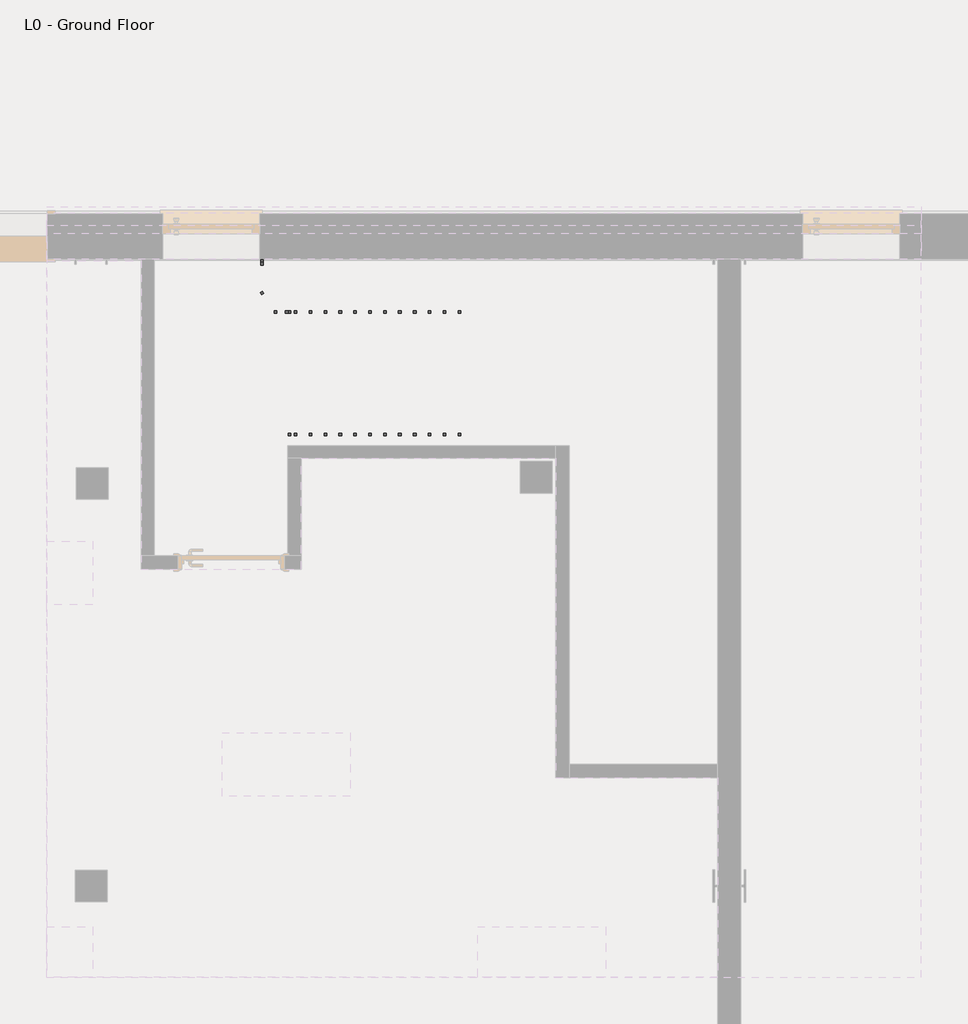
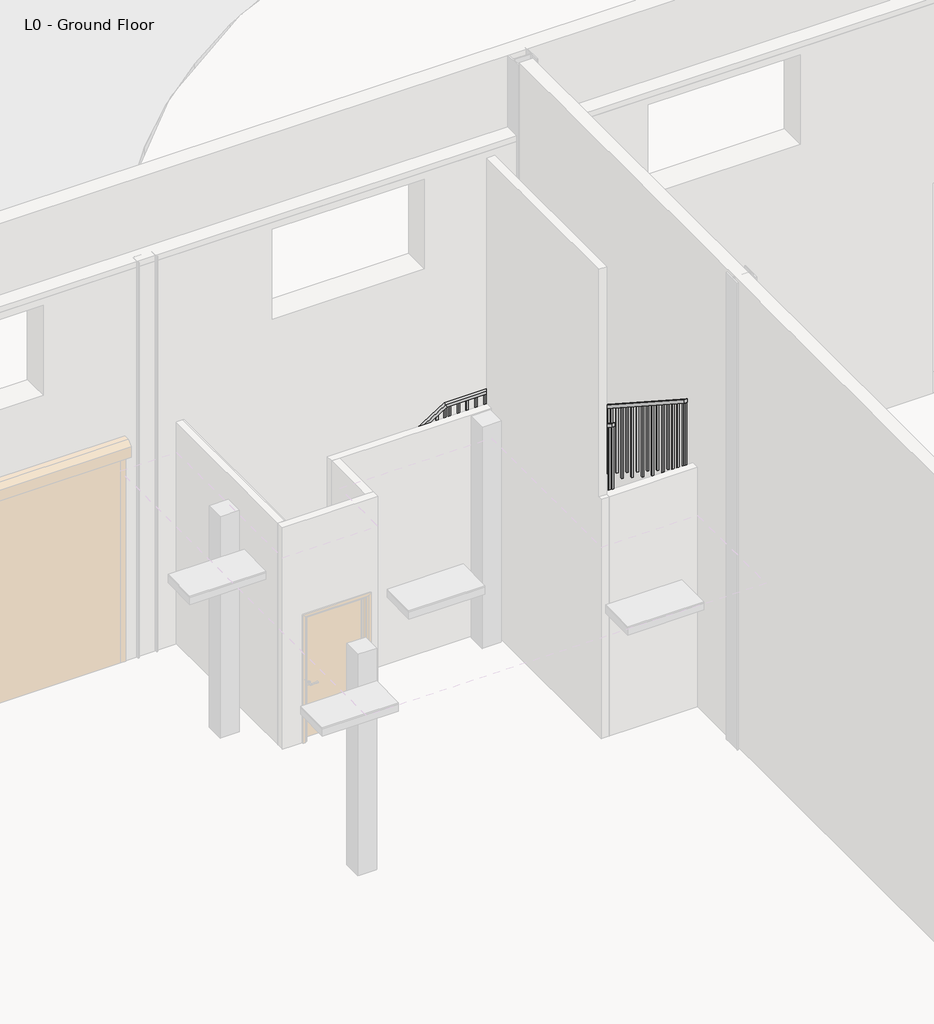
# One storey, part 11 of 14: 3 railings.
"""IFC4 building model written with IfcOpenShell, lengths in millimetres."""

from ifc_helpers import new_model, si_unit, frame, origin, place, context, project, spatial, polyline, outline, extrude, faceted_brep, element, save

model = new_model("IFC4")

# Units and contexts
model_context = context("Model", 3, world=origin())
ifc_project = project(units=[si_unit("LENGTHUNIT", "METRE", prefix="MILLI")], contexts=[model_context])

# Site, building, storey
site = spatial("IfcSite", under=ifc_project)
building = spatial("IfcBuilding", under=site)
storey = spatial("IfcBuildingStorey", under=building, Name="L0 - Ground Floor", Elevation=0.0)

# Railings
placement = place(None, origin())
element("IfcRailing", 1, ObjectType="1100mm", at=placement, inside=storey, context=model_context, shape_type="SolidModel", body=[
    faceted_brep([(6712.9446543, 5212.4222729, 1286.5612648), (6712.9446543, 5212.4222729, 1227.4016553), (6712.9446543, 5162.4222729, 1227.4016553), (6712.9446543, 5162.4222729, 1286.5612648), (9292.9446543, 5212.4222729, 2918.1818182), (9307.4282868, 5212.4222729, 2868.1818182), (9307.4282868, 5162.4222729, 2868.1818182), (9292.9446543, 5162.4222729, 2918.1818182), (9390.9278057, 5212.4222729, 2918.1818182), (9440.9278057, 5212.4222729, 2868.1818182), (9440.9278057, 5162.4222729, 2868.1818182), (9390.9278057, 5162.4222729, 2918.1818182), (9390.9278057, 5212.4222729, 3148.4415584), (9440.9278057, 5212.4222729, 3098.4415584), (9440.9278057, 5162.4222729, 3098.4415584), (9390.9278057, 5162.4222729, 3148.4415584), (9515.9278057, 5212.4222729, 3148.4415584), (9515.9278057, 5212.4222729, 3098.4415584), (9465.9278057, 5162.4222729, 3098.4415584), (9465.9278057, 5162.4222729, 3148.4415584), (9515.9278057, 5087.4222729, 3148.4415584), (9515.9278057, 5072.6126873, 3098.4415584), (9465.9278057, 5072.6126873, 3098.4415584), (9465.9278057, 5087.4222729, 3148.4415584), (9515.9278057, 2082.0222729, 5100.0), (9465.9278057, 2082.0222729, 5100.0), (9465.9278057, 2082.0222729, 5040.383386), (9515.9278057, 2082.0222729, 5040.383386)], [[[0, 1, 2, 3]], [[1, 0, 4, 5]], [[2, 1, 5, 6]], [[3, 2, 6, 7]], [[0, 3, 7, 4]], [[5, 4, 8, 9]], [[6, 5, 9, 10]], [[7, 6, 10, 11]], [[4, 7, 11, 8]], [[9, 8, 12, 13]], [[10, 9, 13, 14]], [[11, 10, 14, 15]], [[8, 11, 15, 12]], [[13, 12, 16, 17]], [[14, 13, 17, 18]], [[15, 14, 18, 19]], [[12, 15, 19, 16]], [[17, 16, 20, 21]], [[18, 17, 21, 22]], [[19, 18, 22, 23]], [[16, 19, 23, 20]], [[24, 25, 26, 27]], [[21, 20, 24, 27]], [[22, 21, 27, 26]], [[23, 22, 26, 25]], [[20, 23, 25, 24]]]),
    extrude(outline(polyline([(2189.9222729, 4970.3184509), (2189.9222729, 3818.1818182), (2164.9222729, 3818.1818182), (2164.9222729, 4986.5522172), (2189.9222729, 4970.3184509)])), frame((9478.4278057, 0.0, 0.0), z_axis=(1.0, 0.0, 0.0), x_axis=(0.0, 1.0, 0.0)), (0.0, 0.0, 1.0), 25.0),
    extrude(outline(polyline([(2329.9222729, 4879.40936), (2329.9222729, 3818.1818182), (2304.9222729, 3818.1818182), (2304.9222729, 4895.6431263), (2329.9222729, 4879.40936)])), frame((9478.4278057, 0.0, 0.0), z_axis=(1.0, 0.0, 0.0), x_axis=(0.0, 1.0, 0.0)), (0.0, 0.0, 1.0), 25.0),
    extrude(outline(polyline([(2469.9222729, 4788.5002691), (2469.9222729, 3636.3636364), (2444.9222729, 3636.3636364), (2444.9222729, 4804.7340354), (2469.9222729, 4788.5002691)])), frame((9478.4278057, 0.0, 0.0), z_axis=(1.0, 0.0, 0.0), x_axis=(0.0, 1.0, 0.0)), (0.0, 0.0, 1.0), 25.0),
    extrude(outline(polyline([(2609.9222729, 4697.5911782), (2609.9222729, 3636.3636364), (2584.9222729, 3636.3636364), (2584.9222729, 4713.8249444), (2609.9222729, 4697.5911782)])), frame((9478.4278057, 0.0, 0.0), z_axis=(1.0, 0.0, 0.0), x_axis=(0.0, 1.0, 0.0)), (0.0, 0.0, 1.0), 25.0),
    extrude(outline(polyline([(2749.9222729, 4606.6820873), (2749.9222729, 3454.5454545), (2724.9222729, 3454.5454545), (2724.9222729, 4622.9158535), (2749.9222729, 4606.6820873)])), frame((9478.4278057, 0.0, 0.0), z_axis=(1.0, 0.0, 0.0), x_axis=(0.0, 1.0, 0.0)), (0.0, 0.0, 1.0), 25.0),
    extrude(outline(polyline([(2889.9222729, 4515.7729964), (2889.9222729, 3454.5454545), (2864.9222729, 3454.5454545), (2864.9222729, 4532.0067626), (2889.9222729, 4515.7729964)])), frame((9478.4278057, 0.0, 0.0), z_axis=(1.0, 0.0, 0.0), x_axis=(0.0, 1.0, 0.0)), (0.0, 0.0, 1.0), 25.0),
    extrude(outline(polyline([(3029.9222729, 4424.8639055), (3029.9222729, 3272.7272727), (3004.9222729, 3272.7272727), (3004.9222729, 4441.0976717), (3029.9222729, 4424.8639055)])), frame((9478.4278057, 0.0, 0.0), z_axis=(1.0, 0.0, 0.0), x_axis=(0.0, 1.0, 0.0)), (0.0, 0.0, 1.0), 25.0),
    extrude(outline(polyline([(3169.9222729, 4333.9548146), (3169.9222729, 3272.7272727), (3144.9222729, 3272.7272727), (3144.9222729, 4350.1885808), (3169.9222729, 4333.9548146)])), frame((9478.4278057, 0.0, 0.0), z_axis=(1.0, 0.0, 0.0), x_axis=(0.0, 1.0, 0.0)), (0.0, 0.0, 1.0), 25.0),
    extrude(outline(polyline([(3309.9222729, 4243.0457237), (3309.9222729, 3090.9090909), (3284.9222729, 3090.9090909), (3284.9222729, 4259.2794899), (3309.9222729, 4243.0457237)])), frame((9478.4278057, 0.0, 0.0), z_axis=(1.0, 0.0, 0.0), x_axis=(0.0, 1.0, 0.0)), (0.0, 0.0, 1.0), 25.0),
    extrude(outline(polyline([(3449.9222729, 4152.1366328), (3449.9222729, 3090.9090909), (3424.9222729, 3090.9090909), (3424.9222729, 4168.370399), (3449.9222729, 4152.1366328)])), frame((9478.4278057, 0.0, 0.0), z_axis=(1.0, 0.0, 0.0), x_axis=(0.0, 1.0, 0.0)), (0.0, 0.0, 1.0), 25.0),
    extrude(outline(polyline([(3589.9222729, 4061.2275418), (3589.9222729, 2909.0909091), (3564.9222729, 2909.0909091), (3564.9222729, 4077.4613081), (3589.9222729, 4061.2275418)])), frame((9478.4278057, 0.0, 0.0), z_axis=(1.0, 0.0, 0.0), x_axis=(0.0, 1.0, 0.0)), (0.0, 0.0, 1.0), 25.0),
    extrude(outline(polyline([(3729.9222729, 3970.3184509), (3729.9222729, 2909.0909091), (3704.9222729, 2909.0909091), (3704.9222729, 3986.5522172), (3729.9222729, 3970.3184509)])), frame((9478.4278057, 0.0, 0.0), z_axis=(1.0, 0.0, 0.0), x_axis=(0.0, 1.0, 0.0)), (0.0, 0.0, 1.0), 25.0),
    extrude(outline(polyline([(3869.9222729, 3879.40936), (3869.9222729, 2727.2727273), (3844.9222729, 2727.2727273), (3844.9222729, 3895.6431263), (3869.9222729, 3879.40936)])), frame((9478.4278057, 0.0, 0.0), z_axis=(1.0, 0.0, 0.0), x_axis=(0.0, 1.0, 0.0)), (0.0, 0.0, 1.0), 25.0),
    extrude(outline(polyline([(4009.9222729, 3788.5002691), (4009.9222729, 2727.2727273), (3984.9222729, 2727.2727273), (3984.9222729, 3804.7340354), (4009.9222729, 3788.5002691)])), frame((9478.4278057, 0.0, 0.0), z_axis=(1.0, 0.0, 0.0), x_axis=(0.0, 1.0, 0.0)), (0.0, 0.0, 1.0), 25.0),
    extrude(outline(polyline([(4149.9222729, 3697.5911782), (4149.9222729, 2545.4545455), (4124.9222729, 2545.4545455), (4124.9222729, 3713.8249444), (4149.9222729, 3697.5911782)])), frame((9478.4278057, 0.0, 0.0), z_axis=(1.0, 0.0, 0.0), x_axis=(0.0, 1.0, 0.0)), (0.0, 0.0, 1.0), 25.0),
    extrude(outline(polyline([(4289.9222729, 3606.6820873), (4289.9222729, 2545.4545455), (4264.9222729, 2545.4545455), (4264.9222729, 3622.9158535), (4289.9222729, 3606.6820873)])), frame((9478.4278057, 0.0, 0.0), z_axis=(1.0, 0.0, 0.0), x_axis=(0.0, 1.0, 0.0)), (0.0, 0.0, 1.0), 25.0),
    extrude(outline(polyline([(4429.9222729, 3515.7729964), (4429.9222729, 2363.6363636), (4404.9222729, 2363.6363636), (4404.9222729, 3532.0067626), (4429.9222729, 3515.7729964)])), frame((9478.4278057, 0.0, 0.0), z_axis=(1.0, 0.0, 0.0), x_axis=(0.0, 1.0, 0.0)), (0.0, 0.0, 1.0), 25.0),
    extrude(outline(polyline([(4569.9222729, 3424.8639055), (4569.9222729, 2363.6363636), (4544.9222729, 2363.6363636), (4544.9222729, 3441.0976717), (4569.9222729, 3424.8639055)])), frame((9478.4278057, 0.0, 0.0), z_axis=(1.0, 0.0, 0.0), x_axis=(0.0, 1.0, 0.0)), (0.0, 0.0, 1.0), 25.0),
    extrude(outline(polyline([(4709.9222729, 3333.9548146), (4709.9222729, 2181.8181818), (4684.9222729, 2181.8181818), (4684.9222729, 3350.1885808), (4709.9222729, 3333.9548146)])), frame((9478.4278057, 0.0, 0.0), z_axis=(1.0, 0.0, 0.0), x_axis=(0.0, 1.0, 0.0)), (0.0, 0.0, 1.0), 25.0),
    extrude(outline(polyline([(4849.9222729, 3243.0457237), (4849.9222729, 2181.8181818), (4824.9222729, 2181.8181818), (4824.9222729, 3259.2794899), (4849.9222729, 3243.0457237)])), frame((9478.4278057, 0.0, 0.0), z_axis=(1.0, 0.0, 0.0), x_axis=(0.0, 1.0, 0.0)), (0.0, 0.0, 1.0), 25.0),
    extrude(outline(polyline([(4989.9222729, 3152.1366328), (4989.9222729, 2000.0), (4964.9222729, 2000.0), (4964.9222729, 3168.370399), (4989.9222729, 3152.1366328)])), frame((9478.4278057, 0.0, 0.0), z_axis=(1.0, 0.0, 0.0), x_axis=(0.0, 1.0, 0.0)), (0.0, 0.0, 1.0), 25.0),
    extrude(outline(polyline([(9478.4278057, 5129.9222729), (9503.4278057, 5129.9222729), (9503.4278057, 5104.9222729), (9478.4278057, 5104.9222729), (9478.4278057, 5129.9222729)])), frame((0.0, 0.0, 2000.0), z_axis=(0.0, 0.0, 1.0), x_axis=(1.0, 0.0, 0.0)), (0.0, 0.0, 1.0), 1098.4415584),
    extrude(outline(polyline([(9350.4446543, 5174.9222729), (9350.4446543, 5199.9222729), (9375.4446543, 5199.9222729), (9375.4446543, 5174.9222729), (9350.4446543, 5174.9222729)])), frame((0.0, 0.0, 1818.1818182), z_axis=(0.0, 0.0, 1.0), x_axis=(1.0, 0.0, 0.0)), (0.0, 0.0, 1.0), 1050.0),
    extrude(outline(polyline([(2768.9036316, 9150.4446543), (1636.3636364, 9150.4446543), (1636.3636364, 9175.4446543), (2784.7139083, 9175.4446543), (2768.9036316, 9150.4446543)])), frame((0.0, 5174.9222729, 0.0), z_axis=(0.0, 1.0, 0.0), x_axis=(0.0, 0.0, 1.0)), (0.0, 0.0, 1.0), 25.0),
    extrude(outline(polyline([(2680.3660822, 9010.4446543), (1636.3636364, 9010.4446543), (1636.3636364, 9035.4446543), (2696.1763589, 9035.4446543), (2680.3660822, 9010.4446543)])), frame((0.0, 5174.9222729, 0.0), z_axis=(0.0, 1.0, 0.0), x_axis=(0.0, 0.0, 1.0)), (0.0, 0.0, 1.0), 25.0),
    extrude(outline(polyline([(2591.8285328, 8870.4446543), (1454.5454545, 8870.4446543), (1454.5454545, 8895.4446543), (2607.6388095, 8895.4446543), (2591.8285328, 8870.4446543)])), frame((0.0, 5174.9222729, 0.0), z_axis=(0.0, 1.0, 0.0), x_axis=(0.0, 0.0, 1.0)), (0.0, 0.0, 1.0), 25.0),
    extrude(outline(polyline([(2503.2909834, 8730.4446543), (1454.5454545, 8730.4446543), (1454.5454545, 8755.4446543), (2519.1012601, 8755.4446543), (2503.2909834, 8730.4446543)])), frame((0.0, 5174.9222729, 0.0), z_axis=(0.0, 1.0, 0.0), x_axis=(0.0, 0.0, 1.0)), (0.0, 0.0, 1.0), 25.0),
    extrude(outline(polyline([(2414.753434, 8590.4446543), (1272.7272727, 8590.4446543), (1272.7272727, 8615.4446543), (2430.5637107, 8615.4446543), (2414.753434, 8590.4446543)])), frame((0.0, 5174.9222729, 0.0), z_axis=(0.0, 1.0, 0.0), x_axis=(0.0, 0.0, 1.0)), (0.0, 0.0, 1.0), 25.0),
    extrude(outline(polyline([(2326.2158846, 8450.4446543), (1272.7272727, 8450.4446543), (1272.7272727, 8475.4446543), (2342.0261613, 8475.4446543), (2326.2158846, 8450.4446543)])), frame((0.0, 5174.9222729, 0.0), z_axis=(0.0, 1.0, 0.0), x_axis=(0.0, 0.0, 1.0)), (0.0, 0.0, 1.0), 25.0),
    extrude(outline(polyline([(2237.6783352, 8310.4446543), (1090.9090909, 8310.4446543), (1090.9090909, 8335.4446543), (2253.4886119, 8335.4446543), (2237.6783352, 8310.4446543)])), frame((0.0, 5174.9222729, 0.0), z_axis=(0.0, 1.0, 0.0), x_axis=(0.0, 0.0, 1.0)), (0.0, 0.0, 1.0), 25.0),
    extrude(outline(polyline([(2149.1407858, 8170.4446543), (1090.9090909, 8170.4446543), (1090.9090909, 8195.4446543), (2164.9510624, 8195.4446543), (2149.1407858, 8170.4446543)])), frame((0.0, 5174.9222729, 0.0), z_axis=(0.0, 1.0, 0.0), x_axis=(0.0, 0.0, 1.0)), (0.0, 0.0, 1.0), 25.0),
    extrude(outline(polyline([(2060.6032364, 8030.4446543), (909.0909091, 8030.4446543), (909.0909091, 8055.4446543), (2076.413513, 8055.4446543), (2060.6032364, 8030.4446543)])), frame((0.0, 5174.9222729, 0.0), z_axis=(0.0, 1.0, 0.0), x_axis=(0.0, 0.0, 1.0)), (0.0, 0.0, 1.0), 25.0),
    extrude(outline(polyline([(1972.065687, 7890.4446543), (909.0909091, 7890.4446543), (909.0909091, 7915.4446543), (1987.8759636, 7915.4446543), (1972.065687, 7890.4446543)])), frame((0.0, 5174.9222729, 0.0), z_axis=(0.0, 1.0, 0.0), x_axis=(0.0, 0.0, 1.0)), (0.0, 0.0, 1.0), 25.0),
    extrude(outline(polyline([(1883.5281375, 7750.4446543), (727.2727273, 7750.4446543), (727.2727273, 7775.4446543), (1899.3384142, 7775.4446543), (1883.5281375, 7750.4446543)])), frame((0.0, 5174.9222729, 0.0), z_axis=(0.0, 1.0, 0.0), x_axis=(0.0, 0.0, 1.0)), (0.0, 0.0, 1.0), 25.0),
    extrude(outline(polyline([(1794.9905881, 7610.4446543), (727.2727273, 7610.4446543), (727.2727273, 7635.4446543), (1810.8008648, 7635.4446543), (1794.9905881, 7610.4446543)])), frame((0.0, 5174.9222729, 0.0), z_axis=(0.0, 1.0, 0.0), x_axis=(0.0, 0.0, 1.0)), (0.0, 0.0, 1.0), 25.0),
    extrude(outline(polyline([(1706.4530387, 7470.4446543), (545.4545455, 7470.4446543), (545.4545455, 7495.4446543), (1722.2633154, 7495.4446543), (1706.4530387, 7470.4446543)])), frame((0.0, 5174.9222729, 0.0), z_axis=(0.0, 1.0, 0.0), x_axis=(0.0, 0.0, 1.0)), (0.0, 0.0, 1.0), 25.0),
    extrude(outline(polyline([(1617.9154893, 7330.4446543), (545.4545455, 7330.4446543), (545.4545455, 7355.4446543), (1633.725766, 7355.4446543), (1617.9154893, 7330.4446543)])), frame((0.0, 5174.9222729, 0.0), z_axis=(0.0, 1.0, 0.0), x_axis=(0.0, 0.0, 1.0)), (0.0, 0.0, 1.0), 25.0),
    extrude(outline(polyline([(1529.3779399, 7190.4446543), (363.6363636, 7190.4446543), (363.6363636, 7215.4446543), (1545.1882166, 7215.4446543), (1529.3779399, 7190.4446543)])), frame((0.0, 5174.9222729, 0.0), z_axis=(0.0, 1.0, 0.0), x_axis=(0.0, 0.0, 1.0)), (0.0, 0.0, 1.0), 25.0),
    extrude(outline(polyline([(1440.8403905, 7050.4446543), (363.6363636, 7050.4446543), (363.6363636, 7075.4446543), (1456.6506672, 7075.4446543), (1440.8403905, 7050.4446543)])), frame((0.0, 5174.9222729, 0.0), z_axis=(0.0, 1.0, 0.0), x_axis=(0.0, 0.0, 1.0)), (0.0, 0.0, 1.0), 25.0),
    extrude(outline(polyline([(1352.3028411, 6910.4446543), (181.8181818, 6910.4446543), (181.8181818, 6935.4446543), (1368.1131178, 6935.4446543), (1352.3028411, 6910.4446543)])), frame((0.0, 5174.9222729, 0.0), z_axis=(0.0, 1.0, 0.0), x_axis=(0.0, 0.0, 1.0)), (0.0, 0.0, 1.0), 25.0),
    extrude(outline(polyline([(1263.7652917, 6770.4446543), (181.8181818, 6770.4446543), (181.8181818, 6795.4446543), (1279.5755684, 6795.4446543), (1263.7652917, 6770.4446543)])), frame((0.0, 5174.9222729, 0.0), z_axis=(0.0, 1.0, 0.0), x_axis=(0.0, 0.0, 1.0)), (0.0, 0.0, 1.0), 25.0),
    extrude(outline(polyline([(9478.4278057, 5199.9222729), (9503.4278057, 5199.9222729), (9503.4278057, 5174.9222729), (9478.4278057, 5174.9222729), (9478.4278057, 5199.9222729)])), frame((0.0, 0.0, 1818.1818182), z_axis=(0.0, 0.0, 1.0), x_axis=(1.0, 0.0, 0.0)), (0.0, 0.0, 1.0), 1280.2597403),
    extrude(outline(polyline([(2851.1170704, 9280.4446543), (1818.1818182, 9280.4446543), (1818.1818182, 9305.4446543), (2866.927347, 9305.4446543), (2851.1170704, 9280.4446543)])), frame((0.0, 5174.9222729, 0.0), z_axis=(0.0, 1.0, 0.0), x_axis=(0.0, 0.0, 1.0)), (0.0, 0.0, 1.0), 25.0),
    extrude(outline(polyline([(2107.0222729, 5024.1496198), (2107.0222729, 3818.1818182), (2082.0222729, 3818.1818182), (2082.0222729, 5040.383386), (2107.0222729, 5024.1496198)])), frame((9478.4278057, 0.0, 0.0), z_axis=(1.0, 0.0, 0.0), x_axis=(0.0, 1.0, 0.0)), (0.0, 0.0, 1.0), 25.0),
    extrude(outline(polyline([(1227.4016553, 6712.9446543), (181.8181818, 6712.9446543), (181.8181818, 6737.9446543), (1243.211932, 6737.9446543), (1227.4016553, 6712.9446543)])), frame((0.0, 5174.9222729, 0.0), z_axis=(0.0, 1.0, 0.0), x_axis=(0.0, 0.0, 1.0)), (0.0, 0.0, 1.0), 25.0),
])
element("IfcRailing", 2, ObjectType="1100mm", at=placement, inside=storey, context=model_context, shape_type="SolidModel", body=[
    faceted_brep([(6712.9446543, 6361.6222729, 1286.5612648), (6712.9446543, 6361.6222729, 1227.4016553), (6712.9446543, 6311.6222729, 1227.4016553), (6712.9446543, 6311.6222729, 1286.5612648), (9292.9446543, 6361.6222729, 2918.1818182), (9307.4282868, 6361.6222729, 2868.1818182), (9307.4282868, 6311.6222729, 2868.1818182), (9292.9446543, 6311.6222729, 2918.1818182), (10665.1278057, 6361.6222729, 2918.1818182), (10665.1278057, 6361.6222729, 2868.1818182), (10615.1278057, 6311.6222729, 2868.1818182), (10615.1278057, 6311.6222729, 2918.1818182), (10665.1278057, 5442.0222729, 2918.1818182), (10665.1278057, 5427.2126873, 2868.1818182), (10615.1278057, 5427.2126873, 2868.1818182), (10615.1278057, 5442.0222729, 2918.1818182), (10665.1278057, 2082.0222729, 5100.0), (10615.1278057, 2082.0222729, 5100.0), (10615.1278057, 2082.0222729, 5040.383386), (10665.1278057, 2082.0222729, 5040.383386)], [[[0, 1, 2, 3]], [[1, 0, 4, 5]], [[2, 1, 5, 6]], [[3, 2, 6, 7]], [[0, 3, 7, 4]], [[5, 4, 8, 9]], [[6, 5, 9, 10]], [[7, 6, 10, 11]], [[4, 7, 11, 8]], [[9, 8, 12, 13]], [[10, 9, 13, 14]], [[11, 10, 14, 15]], [[8, 11, 15, 12]], [[16, 17, 18, 19]], [[13, 12, 16, 19]], [[14, 13, 19, 18]], [[15, 14, 18, 17]], [[12, 15, 17, 16]]]),
    extrude(outline(polyline([(2164.5222729, 3818.1818182), (2139.5222729, 3818.1818182), (2139.5222729, 5003.0457237), (2164.5222729, 4986.8119574), (2164.5222729, 3818.1818182)])), frame((10627.6278057, 0.0, 0.0), z_axis=(1.0, 0.0, 0.0), x_axis=(0.0, 1.0, 0.0)), (0.0, 0.0, 1.0), 25.0),
    extrude(outline(polyline([(2304.5222729, 3818.1818182), (2279.5222729, 3818.1818182), (2279.5222729, 4912.1366328), (2304.5222729, 4895.9028665), (2304.5222729, 3818.1818182)])), frame((10627.6278057, 0.0, 0.0), z_axis=(1.0, 0.0, 0.0), x_axis=(0.0, 1.0, 0.0)), (0.0, 0.0, 1.0), 25.0),
    extrude(outline(polyline([(2444.5222729, 3636.3636364), (2419.5222729, 3636.3636364), (2419.5222729, 4821.2275418), (2444.5222729, 4804.9937756), (2444.5222729, 3636.3636364)])), frame((10627.6278057, 0.0, 0.0), z_axis=(1.0, 0.0, 0.0), x_axis=(0.0, 1.0, 0.0)), (0.0, 0.0, 1.0), 25.0),
    extrude(outline(polyline([(2584.5222729, 3636.3636364), (2559.5222729, 3636.3636364), (2559.5222729, 4730.3184509), (2584.5222729, 4714.0846847), (2584.5222729, 3636.3636364)])), frame((10627.6278057, 0.0, 0.0), z_axis=(1.0, 0.0, 0.0), x_axis=(0.0, 1.0, 0.0)), (0.0, 0.0, 1.0), 25.0),
    extrude(outline(polyline([(2724.5222729, 3454.5454545), (2699.5222729, 3454.5454545), (2699.5222729, 4639.40936), (2724.5222729, 4623.1755938), (2724.5222729, 3454.5454545)])), frame((10627.6278057, 0.0, 0.0), z_axis=(1.0, 0.0, 0.0), x_axis=(0.0, 1.0, 0.0)), (0.0, 0.0, 1.0), 25.0),
    extrude(outline(polyline([(2864.5222729, 3454.5454545), (2839.5222729, 3454.5454545), (2839.5222729, 4548.5002691), (2864.5222729, 4532.2665029), (2864.5222729, 3454.5454545)])), frame((10627.6278057, 0.0, 0.0), z_axis=(1.0, 0.0, 0.0), x_axis=(0.0, 1.0, 0.0)), (0.0, 0.0, 1.0), 25.0),
    extrude(outline(polyline([(3004.5222729, 3272.7272727), (2979.5222729, 3272.7272727), (2979.5222729, 4457.5911782), (3004.5222729, 4441.357412), (3004.5222729, 3272.7272727)])), frame((10627.6278057, 0.0, 0.0), z_axis=(1.0, 0.0, 0.0), x_axis=(0.0, 1.0, 0.0)), (0.0, 0.0, 1.0), 25.0),
    extrude(outline(polyline([(3144.5222729, 3272.7272727), (3119.5222729, 3272.7272727), (3119.5222729, 4366.6820873), (3144.5222729, 4350.4483211), (3144.5222729, 3272.7272727)])), frame((10627.6278057, 0.0, 0.0), z_axis=(1.0, 0.0, 0.0), x_axis=(0.0, 1.0, 0.0)), (0.0, 0.0, 1.0), 25.0),
    extrude(outline(polyline([(3284.5222729, 3090.9090909), (3259.5222729, 3090.9090909), (3259.5222729, 4275.7729964), (3284.5222729, 4259.5392302), (3284.5222729, 3090.9090909)])), frame((10627.6278057, 0.0, 0.0), z_axis=(1.0, 0.0, 0.0), x_axis=(0.0, 1.0, 0.0)), (0.0, 0.0, 1.0), 25.0),
    extrude(outline(polyline([(3424.5222729, 3090.9090909), (3399.5222729, 3090.9090909), (3399.5222729, 4184.8639055), (3424.5222729, 4168.6301392), (3424.5222729, 3090.9090909)])), frame((10627.6278057, 0.0, 0.0), z_axis=(1.0, 0.0, 0.0), x_axis=(0.0, 1.0, 0.0)), (0.0, 0.0, 1.0), 25.0),
    extrude(outline(polyline([(3564.5222729, 2909.0909091), (3539.5222729, 2909.0909091), (3539.5222729, 4093.9548146), (3564.5222729, 4077.7210483), (3564.5222729, 2909.0909091)])), frame((10627.6278057, 0.0, 0.0), z_axis=(1.0, 0.0, 0.0), x_axis=(0.0, 1.0, 0.0)), (0.0, 0.0, 1.0), 25.0),
    extrude(outline(polyline([(3704.5222729, 2909.0909091), (3679.5222729, 2909.0909091), (3679.5222729, 4003.0457237), (3704.5222729, 3986.8119574), (3704.5222729, 2909.0909091)])), frame((10627.6278057, 0.0, 0.0), z_axis=(1.0, 0.0, 0.0), x_axis=(0.0, 1.0, 0.0)), (0.0, 0.0, 1.0), 25.0),
    extrude(outline(polyline([(3844.5222729, 2727.2727273), (3819.5222729, 2727.2727273), (3819.5222729, 3912.1366328), (3844.5222729, 3895.9028665), (3844.5222729, 2727.2727273)])), frame((10627.6278057, 0.0, 0.0), z_axis=(1.0, 0.0, 0.0), x_axis=(0.0, 1.0, 0.0)), (0.0, 0.0, 1.0), 25.0),
    extrude(outline(polyline([(3984.5222729, 2727.2727273), (3959.5222729, 2727.2727273), (3959.5222729, 3821.2275418), (3984.5222729, 3804.9937756), (3984.5222729, 2727.2727273)])), frame((10627.6278057, 0.0, 0.0), z_axis=(1.0, 0.0, 0.0), x_axis=(0.0, 1.0, 0.0)), (0.0, 0.0, 1.0), 25.0),
    extrude(outline(polyline([(4124.5222729, 2545.4545455), (4099.5222729, 2545.4545455), (4099.5222729, 3730.3184509), (4124.5222729, 3714.0846847), (4124.5222729, 2545.4545455)])), frame((10627.6278057, 0.0, 0.0), z_axis=(1.0, 0.0, 0.0), x_axis=(0.0, 1.0, 0.0)), (0.0, 0.0, 1.0), 25.0),
    extrude(outline(polyline([(4264.5222729, 2545.4545455), (4239.5222729, 2545.4545455), (4239.5222729, 3639.40936), (4264.5222729, 3623.1755938), (4264.5222729, 2545.4545455)])), frame((10627.6278057, 0.0, 0.0), z_axis=(1.0, 0.0, 0.0), x_axis=(0.0, 1.0, 0.0)), (0.0, 0.0, 1.0), 25.0),
    extrude(outline(polyline([(4404.5222729, 2363.6363636), (4379.5222729, 2363.6363636), (4379.5222729, 3548.5002691), (4404.5222729, 3532.2665029), (4404.5222729, 2363.6363636)])), frame((10627.6278057, 0.0, 0.0), z_axis=(1.0, 0.0, 0.0), x_axis=(0.0, 1.0, 0.0)), (0.0, 0.0, 1.0), 25.0),
    extrude(outline(polyline([(4544.5222729, 2363.6363636), (4519.5222729, 2363.6363636), (4519.5222729, 3457.5911782), (4544.5222729, 3441.357412), (4544.5222729, 2363.6363636)])), frame((10627.6278057, 0.0, 0.0), z_axis=(1.0, 0.0, 0.0), x_axis=(0.0, 1.0, 0.0)), (0.0, 0.0, 1.0), 25.0),
    extrude(outline(polyline([(4684.5222729, 2181.8181818), (4659.5222729, 2181.8181818), (4659.5222729, 3366.6820873), (4684.5222729, 3350.4483211), (4684.5222729, 2181.8181818)])), frame((10627.6278057, 0.0, 0.0), z_axis=(1.0, 0.0, 0.0), x_axis=(0.0, 1.0, 0.0)), (0.0, 0.0, 1.0), 25.0),
    extrude(outline(polyline([(4824.5222729, 2181.8181818), (4799.5222729, 2181.8181818), (4799.5222729, 3275.7729964), (4824.5222729, 3259.5392302), (4824.5222729, 2181.8181818)])), frame((10627.6278057, 0.0, 0.0), z_axis=(1.0, 0.0, 0.0), x_axis=(0.0, 1.0, 0.0)), (0.0, 0.0, 1.0), 25.0),
    extrude(outline(polyline([(4964.5222729, 2000.0), (4939.5222729, 2000.0), (4939.5222729, 3184.8639055), (4964.5222729, 3168.6301392), (4964.5222729, 2000.0)])), frame((10627.6278057, 0.0, 0.0), z_axis=(1.0, 0.0, 0.0), x_axis=(0.0, 1.0, 0.0)), (0.0, 0.0, 1.0), 25.0),
    extrude(outline(polyline([(5104.5222729, 2000.0), (5079.5222729, 2000.0), (5079.5222729, 3093.9548146), (5104.5222729, 3077.7210483), (5104.5222729, 2000.0)])), frame((10627.6278057, 0.0, 0.0), z_axis=(1.0, 0.0, 0.0), x_axis=(0.0, 1.0, 0.0)), (0.0, 0.0, 1.0), 25.0),
    extrude(outline(polyline([(5244.5222729, 1818.1818182), (5219.5222729, 1818.1818182), (5219.5222729, 3003.0457237), (5244.5222729, 2986.8119574), (5244.5222729, 1818.1818182)])), frame((10627.6278057, 0.0, 0.0), z_axis=(1.0, 0.0, 0.0), x_axis=(0.0, 1.0, 0.0)), (0.0, 0.0, 1.0), 25.0),
    extrude(outline(polyline([(5384.5222729, 1818.1818182), (5359.5222729, 1818.1818182), (5359.5222729, 2912.1366328), (5384.5222729, 2895.9028665), (5384.5222729, 1818.1818182)])), frame((10627.6278057, 0.0, 0.0), z_axis=(1.0, 0.0, 0.0), x_axis=(0.0, 1.0, 0.0)), (0.0, 0.0, 1.0), 25.0),
    extrude(outline(polyline([(10652.6278057, 5579.1222729), (10652.6278057, 5554.1222729), (10627.6278057, 5554.1222729), (10627.6278057, 5579.1222729), (10652.6278057, 5579.1222729)])), frame((0.0, 0.0, 1818.1818182), z_axis=(0.0, 0.0, 1.0), x_axis=(1.0, 0.0, 0.0)), (0.0, 0.0, 1.0), 1050.0),
    extrude(outline(polyline([(10652.6278057, 5719.1222729), (10652.6278057, 5694.1222729), (10627.6278057, 5694.1222729), (10627.6278057, 5719.1222729), (10652.6278057, 5719.1222729)])), frame((0.0, 0.0, 1818.1818182), z_axis=(0.0, 0.0, 1.0), x_axis=(1.0, 0.0, 0.0)), (0.0, 0.0, 1.0), 1050.0),
    extrude(outline(polyline([(10652.6278057, 5859.1222729), (10652.6278057, 5834.1222729), (10627.6278057, 5834.1222729), (10627.6278057, 5859.1222729), (10652.6278057, 5859.1222729)])), frame((0.0, 0.0, 1818.1818182), z_axis=(0.0, 0.0, 1.0), x_axis=(1.0, 0.0, 0.0)), (0.0, 0.0, 1.0), 1050.0),
    extrude(outline(polyline([(10652.6278057, 5999.1222729), (10652.6278057, 5974.1222729), (10627.6278057, 5974.1222729), (10627.6278057, 5999.1222729), (10652.6278057, 5999.1222729)])), frame((0.0, 0.0, 1818.1818182), z_axis=(0.0, 0.0, 1.0), x_axis=(1.0, 0.0, 0.0)), (0.0, 0.0, 1.0), 1050.0),
    extrude(outline(polyline([(10652.6278057, 6139.1222729), (10652.6278057, 6114.1222729), (10627.6278057, 6114.1222729), (10627.6278057, 6139.1222729), (10652.6278057, 6139.1222729)])), frame((0.0, 0.0, 1818.1818182), z_axis=(0.0, 0.0, 1.0), x_axis=(1.0, 0.0, 0.0)), (0.0, 0.0, 1.0), 1050.0),
    extrude(outline(polyline([(10652.6278057, 6279.1222729), (10652.6278057, 6254.1222729), (10627.6278057, 6254.1222729), (10627.6278057, 6279.1222729), (10652.6278057, 6279.1222729)])), frame((0.0, 0.0, 1818.1818182), z_axis=(0.0, 0.0, 1.0), x_axis=(1.0, 0.0, 0.0)), (0.0, 0.0, 1.0), 1050.0),
    extrude(outline(polyline([(10610.4446543, 6349.1222729), (10635.4446543, 6349.1222729), (10635.4446543, 6324.1222729), (10610.4446543, 6324.1222729), (10610.4446543, 6349.1222729)])), frame((0.0, 0.0, 1818.1818182), z_axis=(0.0, 0.0, 1.0), x_axis=(1.0, 0.0, 0.0)), (0.0, 0.0, 1.0), 1050.0),
    extrude(outline(polyline([(10470.4446543, 6349.1222729), (10495.4446543, 6349.1222729), (10495.4446543, 6324.1222729), (10470.4446543, 6324.1222729), (10470.4446543, 6349.1222729)])), frame((0.0, 0.0, 1818.1818182), z_axis=(0.0, 0.0, 1.0), x_axis=(1.0, 0.0, 0.0)), (0.0, 0.0, 1.0), 1050.0),
    extrude(outline(polyline([(10330.4446543, 6349.1222729), (10355.4446543, 6349.1222729), (10355.4446543, 6324.1222729), (10330.4446543, 6324.1222729), (10330.4446543, 6349.1222729)])), frame((0.0, 0.0, 1818.1818182), z_axis=(0.0, 0.0, 1.0), x_axis=(1.0, 0.0, 0.0)), (0.0, 0.0, 1.0), 1050.0),
    extrude(outline(polyline([(10190.4446543, 6349.1222729), (10215.4446543, 6349.1222729), (10215.4446543, 6324.1222729), (10190.4446543, 6324.1222729), (10190.4446543, 6349.1222729)])), frame((0.0, 0.0, 1818.1818182), z_axis=(0.0, 0.0, 1.0), x_axis=(1.0, 0.0, 0.0)), (0.0, 0.0, 1.0), 1050.0),
    extrude(outline(polyline([(10050.4446543, 6349.1222729), (10075.4446543, 6349.1222729), (10075.4446543, 6324.1222729), (10050.4446543, 6324.1222729), (10050.4446543, 6349.1222729)])), frame((0.0, 0.0, 1818.1818182), z_axis=(0.0, 0.0, 1.0), x_axis=(1.0, 0.0, 0.0)), (0.0, 0.0, 1.0), 1050.0),
    extrude(outline(polyline([(9910.4446543, 6349.1222729), (9935.4446543, 6349.1222729), (9935.4446543, 6324.1222729), (9910.4446543, 6324.1222729), (9910.4446543, 6349.1222729)])), frame((0.0, 0.0, 1818.1818182), z_axis=(0.0, 0.0, 1.0), x_axis=(1.0, 0.0, 0.0)), (0.0, 0.0, 1.0), 1050.0),
    extrude(outline(polyline([(9770.4446543, 6349.1222729), (9795.4446543, 6349.1222729), (9795.4446543, 6324.1222729), (9770.4446543, 6324.1222729), (9770.4446543, 6349.1222729)])), frame((0.0, 0.0, 1818.1818182), z_axis=(0.0, 0.0, 1.0), x_axis=(1.0, 0.0, 0.0)), (0.0, 0.0, 1.0), 1050.0),
    extrude(outline(polyline([(9630.4446543, 6349.1222729), (9655.4446543, 6349.1222729), (9655.4446543, 6324.1222729), (9630.4446543, 6324.1222729), (9630.4446543, 6349.1222729)])), frame((0.0, 0.0, 1818.1818182), z_axis=(0.0, 0.0, 1.0), x_axis=(1.0, 0.0, 0.0)), (0.0, 0.0, 1.0), 1050.0),
    extrude(outline(polyline([(9490.4446543, 6349.1222729), (9515.4446543, 6349.1222729), (9515.4446543, 6324.1222729), (9490.4446543, 6324.1222729), (9490.4446543, 6349.1222729)])), frame((0.0, 0.0, 1818.1818182), z_axis=(0.0, 0.0, 1.0), x_axis=(1.0, 0.0, 0.0)), (0.0, 0.0, 1.0), 1050.0),
    extrude(outline(polyline([(9350.4446543, 6349.1222729), (9375.4446543, 6349.1222729), (9375.4446543, 6324.1222729), (9350.4446543, 6324.1222729), (9350.4446543, 6349.1222729)])), frame((0.0, 0.0, 1818.1818182), z_axis=(0.0, 0.0, 1.0), x_axis=(1.0, 0.0, 0.0)), (0.0, 0.0, 1.0), 1050.0),
    extrude(outline(polyline([(1636.3636364, 9150.4446543), (1636.3636364, 9175.4446543), (2784.7139083, 9175.4446543), (2768.9036316, 9150.4446543), (1636.3636364, 9150.4446543)])), frame((0.0, 6324.1222729, 0.0), z_axis=(0.0, 1.0, 0.0), x_axis=(0.0, 0.0, 1.0)), (0.0, 0.0, 1.0), 25.0),
    extrude(outline(polyline([(1636.3636364, 9010.4446543), (1636.3636364, 9035.4446543), (2696.1763589, 9035.4446543), (2680.3660822, 9010.4446543), (1636.3636364, 9010.4446543)])), frame((0.0, 6324.1222729, 0.0), z_axis=(0.0, 1.0, 0.0), x_axis=(0.0, 0.0, 1.0)), (0.0, 0.0, 1.0), 25.0),
    extrude(outline(polyline([(1454.5454545, 8870.4446543), (1454.5454545, 8895.4446543), (2607.6388095, 8895.4446543), (2591.8285328, 8870.4446543), (1454.5454545, 8870.4446543)])), frame((0.0, 6324.1222729, 0.0), z_axis=(0.0, 1.0, 0.0), x_axis=(0.0, 0.0, 1.0)), (0.0, 0.0, 1.0), 25.0),
    extrude(outline(polyline([(1454.5454545, 8730.4446543), (1454.5454545, 8755.4446543), (2519.1012601, 8755.4446543), (2503.2909834, 8730.4446543), (1454.5454545, 8730.4446543)])), frame((0.0, 6324.1222729, 0.0), z_axis=(0.0, 1.0, 0.0), x_axis=(0.0, 0.0, 1.0)), (0.0, 0.0, 1.0), 25.0),
    extrude(outline(polyline([(1272.7272727, 8590.4446543), (1272.7272727, 8615.4446543), (2430.5637107, 8615.4446543), (2414.753434, 8590.4446543), (1272.7272727, 8590.4446543)])), frame((0.0, 6324.1222729, 0.0), z_axis=(0.0, 1.0, 0.0), x_axis=(0.0, 0.0, 1.0)), (0.0, 0.0, 1.0), 25.0),
    extrude(outline(polyline([(1272.7272727, 8450.4446543), (1272.7272727, 8475.4446543), (2342.0261613, 8475.4446543), (2326.2158846, 8450.4446543), (1272.7272727, 8450.4446543)])), frame((0.0, 6324.1222729, 0.0), z_axis=(0.0, 1.0, 0.0), x_axis=(0.0, 0.0, 1.0)), (0.0, 0.0, 1.0), 25.0),
    extrude(outline(polyline([(1090.9090909, 8310.4446543), (1090.9090909, 8335.4446543), (2253.4886119, 8335.4446543), (2237.6783352, 8310.4446543), (1090.9090909, 8310.4446543)])), frame((0.0, 6324.1222729, 0.0), z_axis=(0.0, 1.0, 0.0), x_axis=(0.0, 0.0, 1.0)), (0.0, 0.0, 1.0), 25.0),
    extrude(outline(polyline([(1090.9090909, 8170.4446543), (1090.9090909, 8195.4446543), (2164.9510624, 8195.4446543), (2149.1407858, 8170.4446543), (1090.9090909, 8170.4446543)])), frame((0.0, 6324.1222729, 0.0), z_axis=(0.0, 1.0, 0.0), x_axis=(0.0, 0.0, 1.0)), (0.0, 0.0, 1.0), 25.0),
    extrude(outline(polyline([(909.0909091, 8030.4446543), (909.0909091, 8055.4446543), (2076.413513, 8055.4446543), (2060.6032364, 8030.4446543), (909.0909091, 8030.4446543)])), frame((0.0, 6324.1222729, 0.0), z_axis=(0.0, 1.0, 0.0), x_axis=(0.0, 0.0, 1.0)), (0.0, 0.0, 1.0), 25.0),
    extrude(outline(polyline([(909.0909091, 7890.4446543), (909.0909091, 7915.4446543), (1987.8759636, 7915.4446543), (1972.065687, 7890.4446543), (909.0909091, 7890.4446543)])), frame((0.0, 6324.1222729, 0.0), z_axis=(0.0, 1.0, 0.0), x_axis=(0.0, 0.0, 1.0)), (0.0, 0.0, 1.0), 25.0),
    extrude(outline(polyline([(727.2727273, 7750.4446543), (727.2727273, 7775.4446543), (1899.3384142, 7775.4446543), (1883.5281375, 7750.4446543), (727.2727273, 7750.4446543)])), frame((0.0, 6324.1222729, 0.0), z_axis=(0.0, 1.0, 0.0), x_axis=(0.0, 0.0, 1.0)), (0.0, 0.0, 1.0), 25.0),
    extrude(outline(polyline([(727.2727273, 7610.4446543), (727.2727273, 7635.4446543), (1810.8008648, 7635.4446543), (1794.9905881, 7610.4446543), (727.2727273, 7610.4446543)])), frame((0.0, 6324.1222729, 0.0), z_axis=(0.0, 1.0, 0.0), x_axis=(0.0, 0.0, 1.0)), (0.0, 0.0, 1.0), 25.0),
    extrude(outline(polyline([(545.4545455, 7470.4446543), (545.4545455, 7495.4446543), (1722.2633154, 7495.4446543), (1706.4530387, 7470.4446543), (545.4545455, 7470.4446543)])), frame((0.0, 6324.1222729, 0.0), z_axis=(0.0, 1.0, 0.0), x_axis=(0.0, 0.0, 1.0)), (0.0, 0.0, 1.0), 25.0),
    extrude(outline(polyline([(545.4545455, 7330.4446543), (545.4545455, 7355.4446543), (1633.725766, 7355.4446543), (1617.9154893, 7330.4446543), (545.4545455, 7330.4446543)])), frame((0.0, 6324.1222729, 0.0), z_axis=(0.0, 1.0, 0.0), x_axis=(0.0, 0.0, 1.0)), (0.0, 0.0, 1.0), 25.0),
    extrude(outline(polyline([(363.6363636, 7190.4446543), (363.6363636, 7215.4446543), (1545.1882166, 7215.4446543), (1529.3779399, 7190.4446543), (363.6363636, 7190.4446543)])), frame((0.0, 6324.1222729, 0.0), z_axis=(0.0, 1.0, 0.0), x_axis=(0.0, 0.0, 1.0)), (0.0, 0.0, 1.0), 25.0),
    extrude(outline(polyline([(363.6363636, 7050.4446543), (363.6363636, 7075.4446543), (1456.6506672, 7075.4446543), (1440.8403905, 7050.4446543), (363.6363636, 7050.4446543)])), frame((0.0, 6324.1222729, 0.0), z_axis=(0.0, 1.0, 0.0), x_axis=(0.0, 0.0, 1.0)), (0.0, 0.0, 1.0), 25.0),
    extrude(outline(polyline([(181.8181818, 6910.4446543), (181.8181818, 6935.4446543), (1368.1131178, 6935.4446543), (1352.3028411, 6910.4446543), (181.8181818, 6910.4446543)])), frame((0.0, 6324.1222729, 0.0), z_axis=(0.0, 1.0, 0.0), x_axis=(0.0, 0.0, 1.0)), (0.0, 0.0, 1.0), 25.0),
    extrude(outline(polyline([(181.8181818, 6770.4446543), (181.8181818, 6795.4446543), (1279.5755684, 6795.4446543), (1263.7652917, 6770.4446543), (181.8181818, 6770.4446543)])), frame((0.0, 6324.1222729, 0.0), z_axis=(0.0, 1.0, 0.0), x_axis=(0.0, 0.0, 1.0)), (0.0, 0.0, 1.0), 25.0),
    extrude(outline(polyline([(10652.6278057, 5454.5222729), (10652.6278057, 5429.5222729), (10627.6278057, 5429.5222729), (10627.6278057, 5454.5222729), (10652.6278057, 5454.5222729)])), frame((0.0, 0.0, 1818.1818182), z_axis=(0.0, 0.0, 1.0), x_axis=(1.0, 0.0, 0.0)), (0.0, 0.0, 1.0), 1050.0),
    extrude(outline(polyline([(10627.6278057, 6349.1222729), (10652.6278057, 6349.1222729), (10652.6278057, 6324.1222729), (10627.6278057, 6324.1222729), (10627.6278057, 6349.1222729)])), frame((0.0, 0.0, 1818.1818182), z_axis=(0.0, 0.0, 1.0), x_axis=(1.0, 0.0, 0.0)), (0.0, 0.0, 1.0), 1050.0),
    extrude(outline(polyline([(1818.1818182, 9280.4446543), (1818.1818182, 9305.4446543), (2866.927347, 9305.4446543), (2851.1170704, 9280.4446543), (1818.1818182, 9280.4446543)])), frame((0.0, 6324.1222729, 0.0), z_axis=(0.0, 1.0, 0.0), x_axis=(0.0, 0.0, 1.0)), (0.0, 0.0, 1.0), 25.0),
    extrude(outline(polyline([(2107.0222729, 3818.1818182), (2082.0222729, 3818.1818182), (2082.0222729, 5040.383386), (2107.0222729, 5024.1496198), (2107.0222729, 3818.1818182)])), frame((10627.6278057, 0.0, 0.0), z_axis=(1.0, 0.0, 0.0), x_axis=(0.0, 1.0, 0.0)), (0.0, 0.0, 1.0), 25.0),
    extrude(outline(polyline([(181.8181818, 6712.9446543), (181.8181818, 6737.9446543), (1243.211932, 6737.9446543), (1227.4016553, 6712.9446543), (181.8181818, 6712.9446543)])), frame((0.0, 6324.1222729, 0.0), z_axis=(0.0, 1.0, 0.0), x_axis=(0.0, 0.0, 1.0)), (0.0, 0.0, 1.0), 25.0),
])
element("IfcRailing", 3, ObjectType="1100mm", at=placement, inside=storey, context=model_context, shape_type="SolidModel", body=[
    faceted_brep([(6712.9446543, 6311.6222729, 1280.0), (6712.9446543, 6311.6222729, 1230.0), (6712.9446543, 6361.6222729, 1230.0), (6712.9446543, 6361.6222729, 1280.0), (6579.9304781, 6311.6222729, 1280.0), (6579.9304781, 6311.6222729, 1230.0), (6605.9588306, 6361.6222729, 1230.0), (6605.9588306, 6361.6222729, 1280.0), (6441.7578383, 6508.9532529, 1280.0), (6441.7578383, 6508.9532529, 1230.0), (6491.7578383, 6524.7181924, 1230.0), (6491.7578383, 6524.7181924, 1280.0), (6441.7578383, 6833.7380918, 1280.0), (6491.7578383, 6833.7380918, 1280.0), (6491.7578383, 6833.7380918, 1230.0), (6441.7578383, 6833.7380918, 1230.0)], [[[0, 1, 2, 3]], [[1, 0, 4, 5]], [[2, 1, 5, 6]], [[3, 2, 6, 7]], [[0, 3, 7, 4]], [[5, 4, 8, 9]], [[6, 5, 9, 10]], [[7, 6, 10, 11]], [[4, 7, 11, 8]], [[12, 13, 14, 15]], [[9, 8, 12, 15]], [[10, 9, 15, 14]], [[11, 10, 14, 13]], [[8, 11, 13, 12]]]),
    extrude(outline(polyline([(6479.2578383, 6779.3357226), (6454.2578383, 6779.3357226), (6454.2578383, 6804.3357226), (6479.2578383, 6804.3357226), (6479.2578383, 6779.3357226)])), frame((0.0, 0.0, 180.0), z_axis=(0.0, 0.0, 1.0), x_axis=(1.0, 0.0, 0.0)), (0.0, 0.0, 1.0), 1050.0),
    extrude(outline(polyline([(6484.1669443, 6513.7660275), (6463.6881432, 6499.4266166), (6449.3487323, 6519.9054177), (6469.8275334, 6534.2448287), (6484.1669443, 6513.7660275)])), frame((0.0, 0.0, 180.0), z_axis=(0.0, 0.0, 1.0), x_axis=(1.0, 0.0, 0.0)), (0.0, 0.0, 1.0), 1050.0),
    extrude(outline(polyline([(6605.4446543, 6349.1222729), (6605.4446543, 6324.1222729), (6580.4446543, 6324.1222729), (6580.4446543, 6349.1222729), (6605.4446543, 6349.1222729)])), frame((0.0, 0.0, 180.0), z_axis=(0.0, 0.0, 1.0), x_axis=(1.0, 0.0, 0.0)), (0.0, 0.0, 1.0), 1050.0),
    extrude(outline(polyline([(6479.2578383, 6808.7380918), (6454.2578383, 6808.7380918), (6454.2578383, 6833.7380918), (6479.2578383, 6833.7380918), (6479.2578383, 6808.7380918)])), frame((0.0, 0.0, 180.0), z_axis=(0.0, 0.0, 1.0), x_axis=(1.0, 0.0, 0.0)), (0.0, 0.0, 1.0), 1050.0),
    extrude(outline(polyline([(6712.9446543, 6349.1222729), (6712.9446543, 6324.1222729), (6687.9446543, 6324.1222729), (6687.9446543, 6349.1222729), (6712.9446543, 6349.1222729)])), frame((0.0, 0.0, 180.0), z_axis=(0.0, 0.0, 1.0), x_axis=(1.0, 0.0, 0.0)), (0.0, 0.0, 1.0), 1050.0),
])

save(model, "model.ifc")

# Revit data of these elements
# Type "1100mm"
#   built-in parameter 1008612 = 0.019685 (stored number, unit not read)
#   built-in parameter 1008611 = 0.019685 (stored number, unit not read)
#   built-in parameter 1008609 = 0.902231 (stored number, unit not read)
#   built-in parameter 1008604 = 0.19685 (stored number, unit not read)
#   built-in parameter 1008603 = 0.164042 (stored number, unit not read)
#   Railing Height = 1100 mm
#   built-in parameter 1008630 = 2
#   built-in parameter 1008610 = 2
#   built-in parameter 1008608 = 1
#   built-in parameter 1008618 = Baluster - Square : 25mm
# Elements 1, 2 (IfcRailing, "1100mm")
#   Phase Created = New Construction
# Element 3 (IfcRailing, "1100mm")
#   built-in parameter 1008621 = 0.590551 (stored number, unit not read)
#   Phase Created = New Construction
